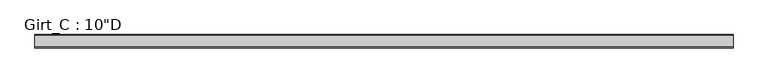
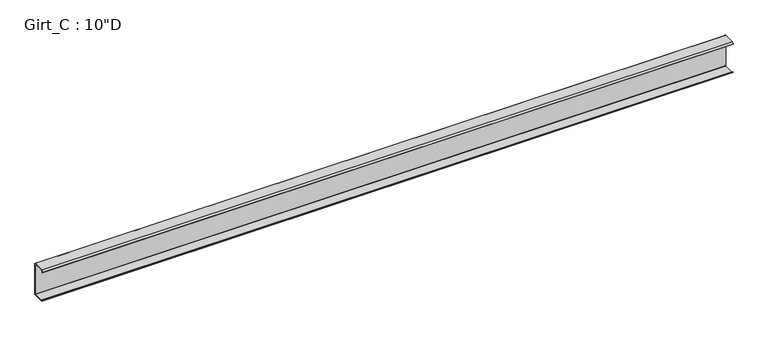
"""IFC4 building model written with IfcOpenShell, lengths in millimetres: beam geometry."""

from ifc_helpers import new_model, si_unit, point, frame, frame_2d, origin, place, context, project, spatial, polyline, circle_curve, trimmed, segment, composite_curve, outline, extrude, source, transform, mapped, element, save


def beam_0183ffdc(model_context):
    return source(origin(), model_context, "Body", "SweptSolid", [
        extrude(outline(composite_curve([segment(polyline([(-87.5109375, 127.0), (-3.3734375, 127.0)]), True, "CONTINUOUS"), segment(trimmed(circle_curve(frame_2d((-3.3734375, 122.2375)), 4.7625), [point((-3.3734375, 127.0))], [point((1.3890625, 122.2375))], False, "CARTESIAN"), True, "CONTINUOUS"), segment(polyline([(1.3890625, 122.2375), (1.3890625, -122.2375)]), True, "CONTINUOUS"), segment(trimmed(circle_curve(frame_2d((-3.3734375, -122.2375)), 4.7625), [point((1.3890625, -122.2375))], [point((-3.3734375, -127.0))], False, "CARTESIAN"), True, "CONTINUOUS"), segment(polyline([(-3.3734375, -127.0), (-87.5109375, -127.0), (-99.7792647, -112.379177), (-97.6510975, -110.5934327), (-86.2154765, -124.221875), (-3.2694106, -124.221875)]), True, "CONTINUOUS"), segment(trimmed(circle_curve(frame_2d((-3.3748024, -122.2389339)), 1.9857399), [point((-3.2694106, -124.221875))], [point((-1.3890625, -122.2389339))], True, "CARTESIAN"), True, "CONTINUOUS"), segment(polyline([(-1.3890625, -122.2389339), (-1.3890625, 122.2381931)]), True, "CONTINUOUS"), segment(trimmed(circle_curve(frame_2d((-3.3741066, 122.2381931)), 1.9850441), [point((-1.3890625, 122.2381931))], [point((-3.3005807, 124.221875))], True, "CARTESIAN"), True, "CONTINUOUS"), segment(polyline([(-3.3005807, 124.221875), (-86.2154765, 124.221875), (-97.6278742, 110.621109), (-99.7560415, 112.4068534), (-87.5109375, 127.0)]), True, "CONTINUOUS")], self_intersect=False)), frame((-2679.319, 0.0, 0.0), z_axis=(1.0, 0.0, 0.0), x_axis=(0.0, 1.0, 0.0)), (0.0, 0.0, 1.0), 5285.613),
    ])


if __name__ == "__main__":
    model = new_model("IFC4")
    model_context = context("Model", 3, world=origin())
    ifc_project = project(units=[si_unit("LENGTHUNIT", "METRE", prefix="MILLI")], contexts=[model_context])
    site = spatial("IfcSite", under=ifc_project)
    building = spatial("IfcBuilding", under=site)
    placement = place(None, origin())
    beam_shape = beam_0183ffdc(model_context)
    element("IfcBeam", 1, ObjectType="Girt_C : 10\"D", at=placement, inside=building, context=model_context, shape_type="MappedRepresentation", body=[
        mapped(beam_shape, transform((0.0, 0.0, 0.0), x_axis=(1.0, 0.0, 0.0), y_axis=(0.0, 1.0, 0.0), z_axis=(0.0, 0.0, 1.0))),
    ])
    save(model, "model.ifc")

# Revit data of these elements
# Type "Girt_C : 10\"D"
#   half leg = 0' - 1 3/4"
#   Web_Thickness = 0' - 0 7/64"
#   Length [instance default] = 10' - 0"
#   Leg_1 = 0' - 3 1/2"
#   Height = 0' - 10"
#   Structural Material [instance default] = none
# Element 1 (IfcBeam, "Girt_C : 10\"D")
#   Structural Material = STRUCTURAL STEEL - SEE STRUCT. DWGS
#   Materials on its faces: "STRUCTURAL STEEL - SEE STRUCT. DWGS"
# Materials
#   "STRUCTURAL STEEL - SEE STRUCT. DWGS": class "Metal", colour RGB 137 146 153, transparency 0, Description = "Steel, mill finish", Cost = 0
